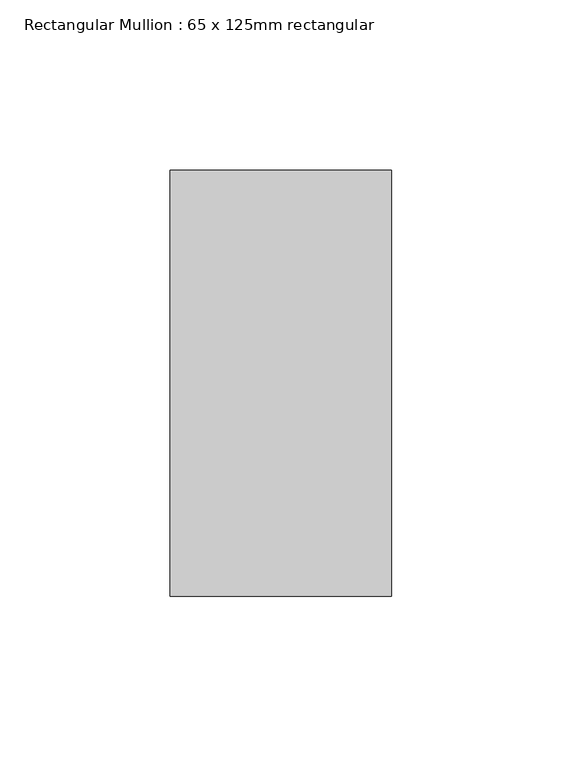
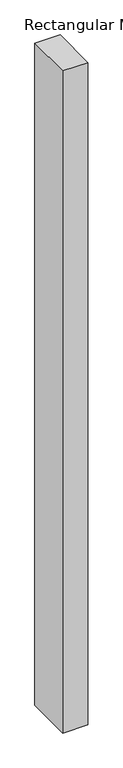
"""IFC4 building model written with IfcOpenShell, lengths in millimetres: member geometry, Rectangular Mullion : 65 x 125mm rectangular."""

from ifc_helpers import new_model, si_unit, frame, origin, place, context, project, spatial, polyline, outline, extrude, source, transform, mapped, element, save


def rectangular_mullion_65_x_125mm_rectangular_567d2977(model_context):
    return source(origin(), model_context, "Body", "SweptSolid", [
        extrude(outline(polyline([(0.0, 62.5), (0.0, -62.5), (-65.0, -62.5), (-65.0, 62.5), (0.0, 62.5)])), frame((0.0, 0.0, -1811.8827626), z_axis=(0.0, 0.0, 1.0), x_axis=(1.0, 0.0, 0.0)), (0.0, 0.0, 1.0), 1811.8827626),
    ])


if __name__ == "__main__":
    model = new_model("IFC4")
    model_context = context("Model", 3, world=origin())
    ifc_project = project(units=[si_unit("LENGTHUNIT", "METRE", prefix="MILLI")], contexts=[model_context])
    site = spatial("IfcSite", under=ifc_project)
    building = spatial("IfcBuilding", under=site)
    placement = place(None, origin())
    rectangular_mullion_65_x_125mm_rectangular_shape = rectangular_mullion_65_x_125mm_rectangular_567d2977(model_context)
    element("IfcMember", 1, ObjectType="Rectangular Mullion : 65 x 125mm rectangular", at=placement, inside=building, context=model_context, shape_type="MappedRepresentation", body=[
        mapped(rectangular_mullion_65_x_125mm_rectangular_shape, transform((0.0, 0.0, 0.0), x_axis=(1.0, 0.0, 0.0), y_axis=(0.0, 1.0, 0.0), z_axis=(0.0, 0.0, 1.0))),
    ])
    save(model, "model.ifc")

# Revit data of these elements
# Type "Rectangular Mullion : 65 x 125mm rectangular"
#   built-in parameter 1007304 = 0.410105 (stored number, unit not read)
#   built-in parameter 1007301 = 0.106627 (stored number, unit not read)
#   built-in parameter 1007300 = 0.106627 (stored number, unit not read)
# Element 1 (IfcMember, "Rectangular Mullion : 65 x 125mm rectangular")
#   Materials on its faces: "Aluminum"
# Materials
#   "Aluminum": class "Metal", colour RGB 244 245 246, transparency 0, Description = "Aluminum 6061", Cost = 0
